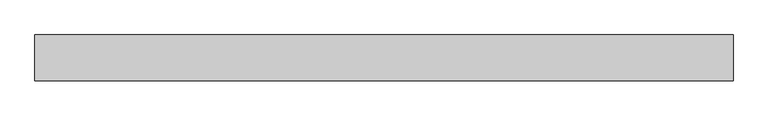
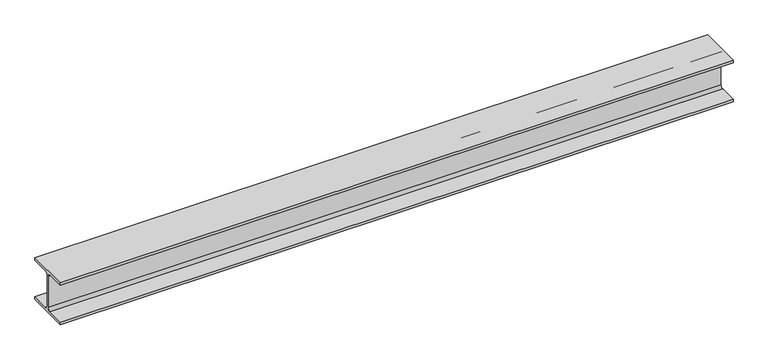
"""IFC4 building model written with IfcOpenShell, lengths in millimetres: beam geometry, 0912_Steel Framing_H-KSD3502 : H_SB_ASB_H-200x200x8x12."""

import ifcopenshell
import ifcopenshell.guid

model = None  # the IFC model being written
_history = None  # IfcOwnerHistory: only IFC2X3 demands one
_inside = {}  # id of a spatial element -> (the spatial element, [elements in it])
_under = {}  # id of a project, library or spatial element -> (it, [spatial elements below it])
_declared = {}  # id of a project -> (the project, [libraries it declares])
_typed = {}  # id of a type object -> (the type object, [elements of that type])
_made_of = {}  # id of a material, layer set ... -> (it, [elements and type objects made of it])


def new_model(schema):
    """Start an empty IFC model of exactly this schema.

    Asked for "IFC4X3", IfcOpenShell would pick the latest addendum, in which some entities
    have other attributes; the version numbers below select the first issue.
    IFC2X3 requires an IfcOwnerHistory on every rooted entity: one is made here for all.
    """
    global model, _history
    if schema == "IFC4X3":
        model = ifcopenshell.file(schema_version=(4, 3, 0, 0))
    else:
        model = ifcopenshell.file(schema=schema)
    _inside.clear()
    _under.clear()
    _declared.clear()
    _typed.clear()
    _made_of.clear()
    _history = None
    if model.schema == "IFC2X3":
        org = make("IfcOrganization", Name="unknown")
        user = make(
            "IfcPersonAndOrganization",
            ThePerson=make("IfcPerson", FamilyName="unknown"),
            TheOrganization=org,
        )
        app = make(
            "IfcApplication",
            ApplicationDeveloper=org,
            Version="unknown",
            ApplicationFullName="unknown",
            ApplicationIdentifier="unknown",
        )
        _history = make(
            "IfcOwnerHistory",
            OwningUser=user,
            OwningApplication=app,
            ChangeAction="ADDED",
            CreationDate=0,
        )
    return model


def make(cls, **values):
    """One entity of the class cls with the attributes given. An attribute that is None is left unset."""
    return model.create_entity(
        cls, **{name: value for name, value in values.items() if value is not None}
    )


def rooted(cls, **values):
    """An entity with a GlobalId (a new one), such as an element, a storey or a relation."""
    return make(cls, GlobalId=ifcopenshell.guid.new(), OwnerHistory=_history, **values)


def si_unit(unit_type, name, prefix=None):
    """IfcSIUnit, for example si_unit("LENGTHUNIT", "METRE", prefix="MILLI")."""
    return make("IfcSIUnit", UnitType=unit_type, Prefix=prefix, Name=name)


def assignment(units):
    """IfcUnitAssignment: the units of a project."""
    return None if units is None else make("IfcUnitAssignment", Units=units)


def point(xyz):
    """IfcCartesianPoint."""
    return None if xyz is None else make("IfcCartesianPoint", Coordinates=xyz)


def direction(xyz):
    """IfcDirection."""
    return None if xyz is None else make("IfcDirection", DirectionRatios=xyz)


def frame(location, z_axis=None, x_axis=None):
    """IfcAxis2Placement3D, a coordinate frame: its origin and axes. An axis left out is left unset."""
    return make(
        "IfcAxis2Placement3D",
        Location=point(location),
        Axis=direction(z_axis),
        RefDirection=direction(x_axis),
    )


def frame_2d(location, x_axis=None):
    """IfcAxis2Placement2D, a coordinate frame in the plane: its origin and x axis."""
    return make(
        "IfcAxis2Placement2D", Location=point(location), RefDirection=direction(x_axis)
    )


def origin():
    """The frame at (0, 0, 0) with its axes left unset."""
    return frame((0.0, 0.0, 0.0))


def place(relative_to, where):
    """IfcLocalPlacement: puts the frame where relative to a parent placement (None: the world)."""
    return make(
        "IfcLocalPlacement", PlacementRelTo=relative_to, RelativePlacement=where
    )


def context(
    kind, dimensions, precision=None, world=None, true_north=None, identifier=None
):
    """IfcGeometricRepresentationContext, for example the 3D "Model" context."""
    return make(
        "IfcGeometricRepresentationContext",
        ContextIdentifier=identifier,
        ContextType=kind,
        CoordinateSpaceDimension=dimensions,
        Precision=precision,
        WorldCoordinateSystem=world,
        TrueNorth=true_north,
    )


def project(units=None, contexts=None):
    """IfcProject with its units and contexts."""
    return rooted(
        "IfcProject",
        Name="project",
        RepresentationContexts=contexts,
        UnitsInContext=assignment(units),
    )


def spatial(cls, under=None, at=None, **own):
    """A site, building, storey or space (cls), placed at a placement, below another one or the project."""
    s = rooted(cls, ObjectPlacement=at, **own)
    if under is not None:
        _under.setdefault(under.id(), (under, []))[1].append(s)
    return s


def polyline(points):
    """IfcPolyline through the points."""
    return make("IfcPolyline", Points=[point(p) for p in points])


def circle_curve(where, radius):
    """IfcCircle in the frame where."""
    return make("IfcCircle", Position=where, Radius=radius)


def trimmed(basis, trim1, trim2, sense, master):
    """IfcTrimmedCurve: the piece of a basis curve between two trims."""
    return make(
        "IfcTrimmedCurve",
        BasisCurve=basis,
        Trim1=trim1,
        Trim2=trim2,
        SenseAgreement=sense,
        MasterRepresentation=master,
    )


def segment(curve, same_sense, transition):
    """IfcCompositeCurveSegment."""
    return make(
        "IfcCompositeCurveSegment",
        Transition=transition,
        SameSense=same_sense,
        ParentCurve=curve,
    )


def composite_curve(segments, self_intersect=None):
    """IfcCompositeCurve: segments joined end to end."""
    return make("IfcCompositeCurve", Segments=segments, SelfIntersect=self_intersect)


def outline(outer, holes=None, kind="AREA"):
    """IfcArbitraryClosedProfileDef: a profile drawn as a closed curve; with holes, ...WithVoids."""
    if holes is None:
        return make("IfcArbitraryClosedProfileDef", ProfileType=kind, OuterCurve=outer)
    return make(
        "IfcArbitraryProfileDefWithVoids",
        ProfileType=kind,
        OuterCurve=outer,
        InnerCurves=holes,
    )


def extrude(swept, where, along, depth):
    """IfcExtrudedAreaSolid: the profile swept, set in the frame where, extruded along a direction by depth."""
    return make(
        "IfcExtrudedAreaSolid",
        SweptArea=swept,
        Position=where,
        ExtrudedDirection=direction(along),
        Depth=depth,
    )


def shape(context_of_items, identifier, shape_type, items):
    """IfcShapeRepresentation: the items that make up one representation, for example the "Body"."""
    return make(
        "IfcShapeRepresentation",
        ContextOfItems=context_of_items,
        RepresentationIdentifier=identifier,
        RepresentationType=shape_type,
        Items=items,
    )


def source(mapping_origin, context_of_items, identifier, shape_type, items):
    """IfcRepresentationMap: a shape defined once, which mapped items show again and again."""
    return make(
        "IfcRepresentationMap",
        MappingOrigin=mapping_origin,
        MappedRepresentation=shape(context_of_items, identifier, shape_type, items),
    )


def transform(
    local_origin,
    x_axis=None,
    y_axis=None,
    z_axis=None,
    scale=None,
    scale2=None,
    scale3=None,
    uniform=True,
):
    """IfcCartesianTransformationOperator3D, or its non-uniform kind. x_axis, y_axis, z_axis: its Axis1, 2, 3."""
    if uniform:
        return make(
            "IfcCartesianTransformationOperator3D",
            Axis1=direction(x_axis),
            Axis2=direction(y_axis),
            LocalOrigin=point(local_origin),
            Scale=scale,
            Axis3=direction(z_axis),
        )
    return make(
        "IfcCartesianTransformationOperator3DnonUniform",
        Axis1=direction(x_axis),
        Axis2=direction(y_axis),
        LocalOrigin=point(local_origin),
        Scale=scale,
        Axis3=direction(z_axis),
        Scale2=scale2,
        Scale3=scale3,
    )


def mapped(mapping_source, mapping_target):
    """IfcMappedItem: shows the shape of a source again, moved by a transform."""
    return make(
        "IfcMappedItem", MappingSource=mapping_source, MappingTarget=mapping_target
    )


def made_of(thing, what):
    """Note that an element or type object is made of a material, layer set ...; save() writes the relation."""
    if what is not None:
        _made_of.setdefault(what.id(), (what, []))[1].append(thing)
    return thing


def element(
    cls,
    number,
    at=None,
    inside=None,
    cuts=None,
    type_object=None,
    material=None,
    context=None,
    identifier="Body",
    shape_type=None,
    held_by="IfcProductDefinitionShape",
    body=None,
    shapes=None,
    **own,
):
    """One element of the class cls, such as IfcWall. Its Tag is "e" and its number.

    at: its placement. inside: the storey or other place that contains it. cuts: it is an
    opening in that element (IfcRelVoidsElement). A single representation is given by context,
    identifier, shape_type and body (its items); several are given by shapes. held_by: the class
    of the entity that holds the representations. save() writes the other relations.
    """
    e = rooted(cls, Tag="e%d" % number, ObjectPlacement=at, **own)
    if body is not None:
        shapes = [shape(context, identifier, shape_type, body)]
    if shapes is not None:
        e.Representation = make(held_by, Representations=shapes)
    if inside is not None:
        _inside.setdefault(inside.id(), (inside, []))[1].append(e)
    if cuts is not None:
        rooted(
            "IfcRelVoidsElement", RelatingBuildingElement=cuts, RelatedOpeningElement=e
        )
    if type_object is not None:
        _typed.setdefault(type_object.id(), (type_object, []))[1].append(e)
    return made_of(e, material)


def aggregate(whole, parts):
    """IfcRelAggregates: a whole, such as a stair, and the parts it consists of."""
    return rooted("IfcRelAggregates", RelatingObject=whole, RelatedObjects=parts)


def save(model, path):
    """Write the relations noted so far, then the file.

    IfcRelAggregates (storeys below a building ...), IfcRelContainedInSpatialStructure (elements
    in a storey), IfcRelDefinesByType, IfcRelAssociatesMaterial and IfcRelDeclares: one each for
    every whole, place, type object, material and project.
    """
    for whole, parts in _under.values():
        aggregate(whole, parts)
    for where, things in _inside.values():
        rooted(
            "IfcRelContainedInSpatialStructure",
            RelatedElements=things,
            RelatingStructure=where,
        )
    for kind, things in _typed.values():
        rooted("IfcRelDefinesByType", RelatedObjects=things, RelatingType=kind)
    for what, things in _made_of.values():
        rooted("IfcRelAssociatesMaterial", RelatedObjects=things, RelatingMaterial=what)
    for by, libraries in _declared.values():
        rooted("IfcRelDeclares", RelatingContext=by, RelatedDefinitions=libraries)
    model.write(path)


def beam_a4cbd311(model_context):
    return source(origin(), model_context, "Body", "SweptSolid", [
        extrude(outline(composite_curve([segment(polyline([(100.0, -88.0), (100.0, -100.0), (-100.0, -100.0), (-100.0, -88.0), (-17.0, -88.0)]), True, "CONTINUOUS"), segment(trimmed(circle_curve(frame_2d((-17.0, -75.0)), 13.0), [point((-17.0, -88.0))], [point((-4.0, -75.0))], True, "CARTESIAN"), True, "CONTINUOUS"), segment(polyline([(-4.0, -75.0), (-4.0, 75.0)]), True, "CONTINUOUS"), segment(trimmed(circle_curve(frame_2d((-17.0, 75.0)), 13.0), [point((-4.0, 75.0))], [point((-17.0, 88.0))], True, "CARTESIAN"), True, "CONTINUOUS"), segment(polyline([(-17.0, 88.0), (-100.0, 88.0), (-100.0, 100.0), (100.0, 100.0), (100.0, 88.0), (17.0, 88.0)]), True, "CONTINUOUS"), segment(trimmed(circle_curve(frame_2d((17.0, 75.0)), 13.0), [point((17.0, 88.0))], [point((4.0, 75.0))], True, "CARTESIAN"), True, "CONTINUOUS"), segment(polyline([(4.0, 75.0), (4.0, -75.0)]), True, "CONTINUOUS"), segment(trimmed(circle_curve(frame_2d((17.0, -75.0)), 13.0), [point((4.0, -75.0))], [point((17.0, -88.0))], True, "CARTESIAN"), True, "CONTINUOUS"), segment(polyline([(17.0, -88.0), (100.0, -88.0)]), True, "CONTINUOUS")], self_intersect=False)), frame((-1342.7433978, 0.0, 0.0), z_axis=(1.0, 0.0, 0.0), x_axis=(0.0, 1.0, 0.0)), (0.0, 0.0, 1.0), 3052.6875076),
    ])


if __name__ == "__main__":
    model = new_model("IFC4")
    model_context = context("Model", 3, world=origin())
    ifc_project = project(units=[si_unit("LENGTHUNIT", "METRE", prefix="MILLI")], contexts=[model_context])
    site = spatial("IfcSite", under=ifc_project)
    building = spatial("IfcBuilding", under=site)
    placement = place(None, origin())
    beam_shape = beam_a4cbd311(model_context)
    element("IfcBeam", 1, ObjectType="0912_Steel Framing_H-KSD3502 : H_SB_ASB_H-200x200x8x12", at=placement, inside=building, context=model_context, shape_type="MappedRepresentation", body=[
        mapped(beam_shape, transform((0.0, 0.0, 0.0), x_axis=(1.0, 0.0, 0.0), y_axis=(0.0, 1.0, 0.0), z_axis=(0.0, 0.0, 1.0))),
    ])
    save(model, "model.ifc")

# Revit data of these elements
# Type "0912_Steel Framing_H-KSD3502 : H_SB_ASB_H-200x200x8x12"
#   H_WM Code_1 = "S01AA002-00001 | Main Steel Structure Fabrication Work | Shelter/Building | Medium Steel - Standard (90KG/M>Weight≥30KG/M) | Material: (   )"
#   H_WM Code_2 = "S03AA028-00001 | Main Steel Structure Erection Work | Shelter/Building | Medium Steel (90KG/M>Weight≥30KG/M) | Material: (   )"
#   H_WM Code_3 = "S01AA010-00001 | Main Steel Structure Fabrication Work | Shelter/Building | Steel Painting/Coating | for Non-Fireproofed Steel Surface, Surface Preparation, Primer, Second & Final Coat | Material: (   )"
#   H_Q'ty Cal Type Tag = "SB-Q2"
#   Width = 20.0 cm
#   Web Thickness = 0.8 cm
#   Web Fillet = 1.3 cm
#   Warping Constant = 141000.0 cm⁶
#   W = 0
#   Torsional Moment of Inertia = 26.2485 cm⁴
#   Section Area = 63.53 cm²
#   Plastic Modulus weak axis = 244.0 cm³
#   Plastic Modulus strong axis = 525.0 cm³
#   Perimeter = 1.16 m²/m
#   Nominal Weight = 49.90 kgf/m
#   Moment of Inertia weak axis = 1600.00 cm⁴
#   Moment of Inertia strong axis = 4720.00 cm⁴
#   Height = 20.0 cm
#   Flange Thickness = 1.2 cm
#   Elastic Modulus weak axis = 160.0 cm³
#   Elastic Modulus strong axis = 472.0 cm³
#   Centroid Vertical = 10.0 cm
#   Centroid Horizontal = 10.0 cm
#   Ix = 47200000
#   Length [instance default] = 1.5240 m
#   Zx = 525000
#   b = 0.2000 m
#   h = 0.2000 m
#   r = 0.0130 m
#   s = 0.0080 m
#   t = 0.0120 m
#   A = 0.006353 m²
#   Structural Material [instance default] = Steel, 45-345
#   Assembly Code = ""
# Element 1 (IfcBeam, "0912_Steel Framing_H-KSD3502 : H_SB_ASB_H-200x200x8x12")
#   Structural Material = none
# Materials
#   "Steel, 45-345": class "Metal", colour RGB 189 187 185, transparency 0, Description = "Steel 345 MPa", Cost = 0
